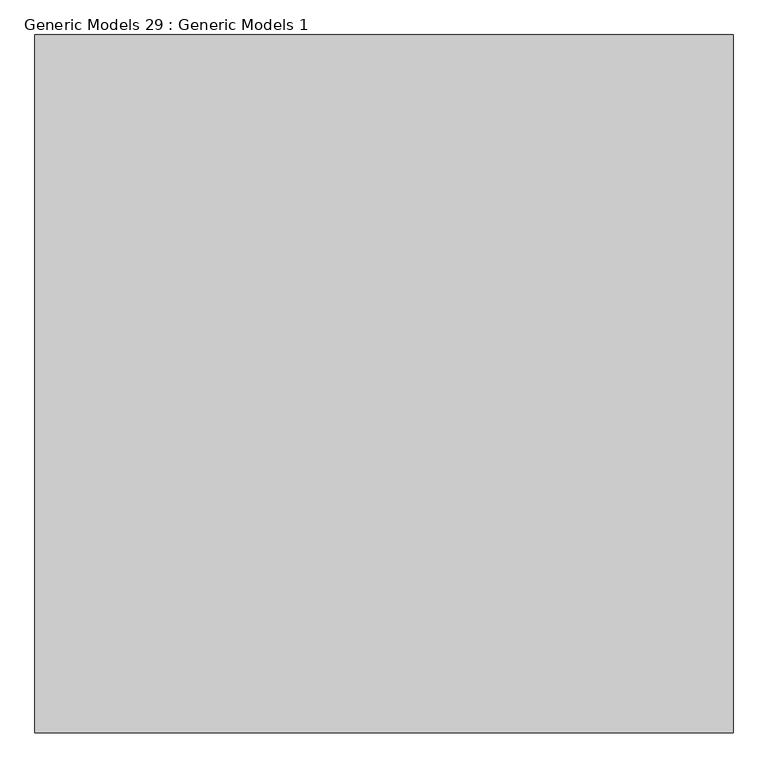
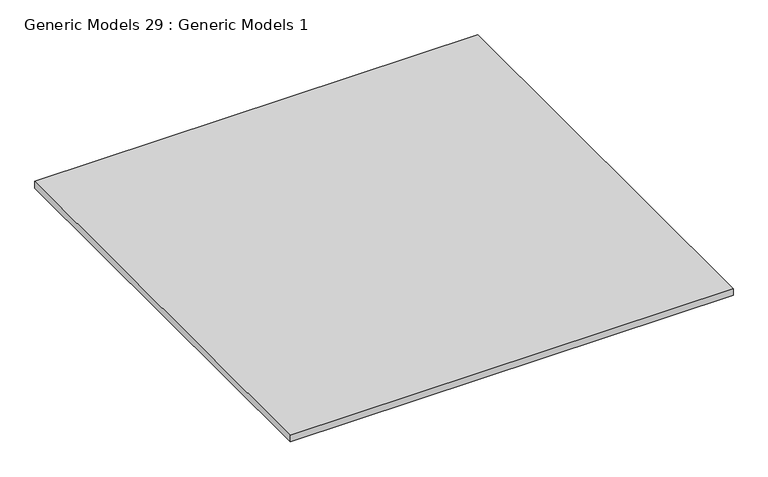
"""IFC4 building model written with IfcOpenShell, lengths in millimetres: proxy geometry, Generic Models 29 : Generic Models 1."""

import ifcopenshell
import ifcopenshell.guid

model = None  # the IFC model being written
_history = None  # IfcOwnerHistory: only IFC2X3 demands one
_inside = {}  # id of a spatial element -> (the spatial element, [elements in it])
_under = {}  # id of a project, library or spatial element -> (it, [spatial elements below it])
_declared = {}  # id of a project -> (the project, [libraries it declares])
_typed = {}  # id of a type object -> (the type object, [elements of that type])
_made_of = {}  # id of a material, layer set ... -> (it, [elements and type objects made of it])


def new_model(schema):
    """Start an empty IFC model of exactly this schema.

    Asked for "IFC4X3", IfcOpenShell would pick the latest addendum, in which some entities
    have other attributes; the version numbers below select the first issue.
    IFC2X3 requires an IfcOwnerHistory on every rooted entity: one is made here for all.
    """
    global model, _history
    if schema == "IFC4X3":
        model = ifcopenshell.file(schema_version=(4, 3, 0, 0))
    else:
        model = ifcopenshell.file(schema=schema)
    _inside.clear()
    _under.clear()
    _declared.clear()
    _typed.clear()
    _made_of.clear()
    _history = None
    if model.schema == "IFC2X3":
        org = make("IfcOrganization", Name="unknown")
        user = make(
            "IfcPersonAndOrganization",
            ThePerson=make("IfcPerson", FamilyName="unknown"),
            TheOrganization=org,
        )
        app = make(
            "IfcApplication",
            ApplicationDeveloper=org,
            Version="unknown",
            ApplicationFullName="unknown",
            ApplicationIdentifier="unknown",
        )
        _history = make(
            "IfcOwnerHistory",
            OwningUser=user,
            OwningApplication=app,
            ChangeAction="ADDED",
            CreationDate=0,
        )
    return model


def make(cls, **values):
    """One entity of the class cls with the attributes given. An attribute that is None is left unset."""
    return model.create_entity(
        cls, **{name: value for name, value in values.items() if value is not None}
    )


def rooted(cls, **values):
    """An entity with a GlobalId (a new one), such as an element, a storey or a relation."""
    return make(cls, GlobalId=ifcopenshell.guid.new(), OwnerHistory=_history, **values)


def si_unit(unit_type, name, prefix=None):
    """IfcSIUnit, for example si_unit("LENGTHUNIT", "METRE", prefix="MILLI")."""
    return make("IfcSIUnit", UnitType=unit_type, Prefix=prefix, Name=name)


def assignment(units):
    """IfcUnitAssignment: the units of a project."""
    return None if units is None else make("IfcUnitAssignment", Units=units)


def point(xyz):
    """IfcCartesianPoint."""
    return None if xyz is None else make("IfcCartesianPoint", Coordinates=xyz)


def direction(xyz):
    """IfcDirection."""
    return None if xyz is None else make("IfcDirection", DirectionRatios=xyz)


def frame(location, z_axis=None, x_axis=None):
    """IfcAxis2Placement3D, a coordinate frame: its origin and axes. An axis left out is left unset."""
    return make(
        "IfcAxis2Placement3D",
        Location=point(location),
        Axis=direction(z_axis),
        RefDirection=direction(x_axis),
    )


def origin():
    """The frame at (0, 0, 0) with its axes left unset."""
    return frame((0.0, 0.0, 0.0))


def place(relative_to, where):
    """IfcLocalPlacement: puts the frame where relative to a parent placement (None: the world)."""
    return make(
        "IfcLocalPlacement", PlacementRelTo=relative_to, RelativePlacement=where
    )


def context(
    kind, dimensions, precision=None, world=None, true_north=None, identifier=None
):
    """IfcGeometricRepresentationContext, for example the 3D "Model" context."""
    return make(
        "IfcGeometricRepresentationContext",
        ContextIdentifier=identifier,
        ContextType=kind,
        CoordinateSpaceDimension=dimensions,
        Precision=precision,
        WorldCoordinateSystem=world,
        TrueNorth=true_north,
    )


def project(units=None, contexts=None):
    """IfcProject with its units and contexts."""
    return rooted(
        "IfcProject",
        Name="project",
        RepresentationContexts=contexts,
        UnitsInContext=assignment(units),
    )


def spatial(cls, under=None, at=None, **own):
    """A site, building, storey or space (cls), placed at a placement, below another one or the project."""
    s = rooted(cls, ObjectPlacement=at, **own)
    if under is not None:
        _under.setdefault(under.id(), (under, []))[1].append(s)
    return s


def polyline(points):
    """IfcPolyline through the points."""
    return make("IfcPolyline", Points=[point(p) for p in points])


def outline(outer, holes=None, kind="AREA"):
    """IfcArbitraryClosedProfileDef: a profile drawn as a closed curve; with holes, ...WithVoids."""
    if holes is None:
        return make("IfcArbitraryClosedProfileDef", ProfileType=kind, OuterCurve=outer)
    return make(
        "IfcArbitraryProfileDefWithVoids",
        ProfileType=kind,
        OuterCurve=outer,
        InnerCurves=holes,
    )


def extrude(swept, where, along, depth):
    """IfcExtrudedAreaSolid: the profile swept, set in the frame where, extruded along a direction by depth."""
    return make(
        "IfcExtrudedAreaSolid",
        SweptArea=swept,
        Position=where,
        ExtrudedDirection=direction(along),
        Depth=depth,
    )


def shape(context_of_items, identifier, shape_type, items):
    """IfcShapeRepresentation: the items that make up one representation, for example the "Body"."""
    return make(
        "IfcShapeRepresentation",
        ContextOfItems=context_of_items,
        RepresentationIdentifier=identifier,
        RepresentationType=shape_type,
        Items=items,
    )


def source(mapping_origin, context_of_items, identifier, shape_type, items):
    """IfcRepresentationMap: a shape defined once, which mapped items show again and again."""
    return make(
        "IfcRepresentationMap",
        MappingOrigin=mapping_origin,
        MappedRepresentation=shape(context_of_items, identifier, shape_type, items),
    )


def transform(
    local_origin,
    x_axis=None,
    y_axis=None,
    z_axis=None,
    scale=None,
    scale2=None,
    scale3=None,
    uniform=True,
):
    """IfcCartesianTransformationOperator3D, or its non-uniform kind. x_axis, y_axis, z_axis: its Axis1, 2, 3."""
    if uniform:
        return make(
            "IfcCartesianTransformationOperator3D",
            Axis1=direction(x_axis),
            Axis2=direction(y_axis),
            LocalOrigin=point(local_origin),
            Scale=scale,
            Axis3=direction(z_axis),
        )
    return make(
        "IfcCartesianTransformationOperator3DnonUniform",
        Axis1=direction(x_axis),
        Axis2=direction(y_axis),
        LocalOrigin=point(local_origin),
        Scale=scale,
        Axis3=direction(z_axis),
        Scale2=scale2,
        Scale3=scale3,
    )


def mapped(mapping_source, mapping_target):
    """IfcMappedItem: shows the shape of a source again, moved by a transform."""
    return make(
        "IfcMappedItem", MappingSource=mapping_source, MappingTarget=mapping_target
    )


def made_of(thing, what):
    """Note that an element or type object is made of a material, layer set ...; save() writes the relation."""
    if what is not None:
        _made_of.setdefault(what.id(), (what, []))[1].append(thing)
    return thing


def element(
    cls,
    number,
    at=None,
    inside=None,
    cuts=None,
    type_object=None,
    material=None,
    context=None,
    identifier="Body",
    shape_type=None,
    held_by="IfcProductDefinitionShape",
    body=None,
    shapes=None,
    **own,
):
    """One element of the class cls, such as IfcWall. Its Tag is "e" and its number.

    at: its placement. inside: the storey or other place that contains it. cuts: it is an
    opening in that element (IfcRelVoidsElement). A single representation is given by context,
    identifier, shape_type and body (its items); several are given by shapes. held_by: the class
    of the entity that holds the representations. save() writes the other relations.
    """
    e = rooted(cls, Tag="e%d" % number, ObjectPlacement=at, **own)
    if body is not None:
        shapes = [shape(context, identifier, shape_type, body)]
    if shapes is not None:
        e.Representation = make(held_by, Representations=shapes)
    if inside is not None:
        _inside.setdefault(inside.id(), (inside, []))[1].append(e)
    if cuts is not None:
        rooted(
            "IfcRelVoidsElement", RelatingBuildingElement=cuts, RelatedOpeningElement=e
        )
    if type_object is not None:
        _typed.setdefault(type_object.id(), (type_object, []))[1].append(e)
    return made_of(e, material)


def aggregate(whole, parts):
    """IfcRelAggregates: a whole, such as a stair, and the parts it consists of."""
    return rooted("IfcRelAggregates", RelatingObject=whole, RelatedObjects=parts)


def save(model, path):
    """Write the relations noted so far, then the file.

    IfcRelAggregates (storeys below a building ...), IfcRelContainedInSpatialStructure (elements
    in a storey), IfcRelDefinesByType, IfcRelAssociatesMaterial and IfcRelDeclares: one each for
    every whole, place, type object, material and project.
    """
    for whole, parts in _under.values():
        aggregate(whole, parts)
    for where, things in _inside.values():
        rooted(
            "IfcRelContainedInSpatialStructure",
            RelatedElements=things,
            RelatingStructure=where,
        )
    for kind, things in _typed.values():
        rooted("IfcRelDefinesByType", RelatedObjects=things, RelatingType=kind)
    for what, things in _made_of.values():
        rooted("IfcRelAssociatesMaterial", RelatedObjects=things, RelatingMaterial=what)
    for by, libraries in _declared.values():
        rooted("IfcRelDeclares", RelatingContext=by, RelatedDefinitions=libraries)
    model.write(path)


def generic_models_29_generic_models_1_59087225(model_context):
    return source(origin(), model_context, "Body", "SweptSolid", [
        extrude(outline(polyline([(50347.5625, 1219.2), (50347.5625, 0.0), (49128.3625, 0.0), (49128.3625, 1219.2), (50347.5625, 1219.2)])), frame((0.0, 0.0, 5647.53125), z_axis=(0.0, 0.0, 1.0), x_axis=(1.0, 0.0, 0.0)), (0.0, 0.0, 1.0), 19.05),
    ])


if __name__ == "__main__":
    model = new_model("IFC4")
    model_context = context("Model", 3, world=origin())
    ifc_project = project(units=[si_unit("LENGTHUNIT", "METRE", prefix="MILLI")], contexts=[model_context])
    site = spatial("IfcSite", under=ifc_project)
    building = spatial("IfcBuilding", under=site)
    placement = place(None, origin())
    generic_models_29_generic_models_1_shape = generic_models_29_generic_models_1_59087225(model_context)
    element("IfcBuildingElementProxy", 1, Name="Generic Models 29 : Generic Models 1", ObjectType="Generic Models 29 : Generic Models 1", at=placement, inside=building, context=model_context, shape_type="MappedRepresentation", body=[
        mapped(generic_models_29_generic_models_1_shape, transform((0.0, 0.0, 0.0), x_axis=(1.0, 0.0, 0.0), y_axis=(0.0, 1.0, 0.0), z_axis=(0.0, 0.0, 1.0))),
    ])
    save(model, "model.ifc")

# Revit data of these elements
# Element 1 (IfcBuildingElementProxy, "Generic Models 29 : Generic Models 1")
#   Materials on its faces: "SUBSTRATE AS SCHEDULED"
# Materials
#   "SUBSTRATE AS SCHEDULED": class "Unassigned", colour RGB 196 177 123, transparency 0, Cost = 0
